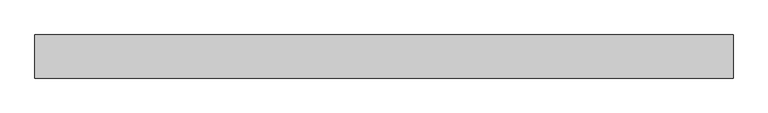
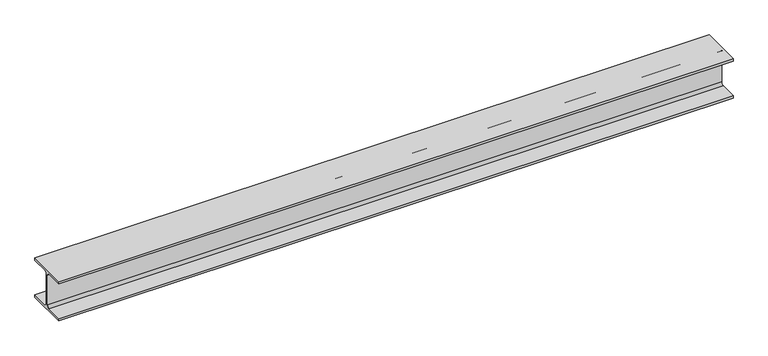
"""IFC4 building model written with IfcOpenShell, lengths in millimetres: beam geometry, 0912_Steel Framing_H-KSD3502 : H_SB_ASB_H-200x200x8x12."""

from ifc_helpers import new_model, si_unit, point, frame, frame_2d, origin, place, context, project, spatial, polyline, circle_curve, trimmed, segment, composite_curve, outline, extrude, source, transform, mapped, element, save


def beam_a703e86a(model_context):
    return source(origin(), model_context, "Body", "SweptSolid", [
        extrude(outline(composite_curve([segment(polyline([(100.0, -88.0), (100.0, -100.0), (-100.0, -100.0), (-100.0, -88.0), (-17.0, -88.0)]), True, "CONTINUOUS"), segment(trimmed(circle_curve(frame_2d((-17.0, -75.0)), 13.0), [point((-17.0, -88.0))], [point((-4.0, -75.0))], True, "CARTESIAN"), True, "CONTINUOUS"), segment(polyline([(-4.0, -75.0), (-4.0, 75.0)]), True, "CONTINUOUS"), segment(trimmed(circle_curve(frame_2d((-17.0, 75.0)), 13.0), [point((-4.0, 75.0))], [point((-17.0, 88.0))], True, "CARTESIAN"), True, "CONTINUOUS"), segment(polyline([(-17.0, 88.0), (-100.0, 88.0), (-100.0, 100.0), (100.0, 100.0), (100.0, 88.0), (17.0, 88.0)]), True, "CONTINUOUS"), segment(trimmed(circle_curve(frame_2d((17.0, 75.0)), 13.0), [point((17.0, 88.0))], [point((4.0, 75.0))], True, "CARTESIAN"), True, "CONTINUOUS"), segment(polyline([(4.0, 75.0), (4.0, -75.0)]), True, "CONTINUOUS"), segment(trimmed(circle_curve(frame_2d((17.0, -75.0)), 13.0), [point((4.0, -75.0))], [point((17.0, -88.0))], True, "CARTESIAN"), True, "CONTINUOUS"), segment(polyline([(17.0, -88.0), (100.0, -88.0)]), True, "CONTINUOUS")], self_intersect=False)), frame((-1414.4668129, 0.0, 0.0), z_axis=(1.0, 0.0, 0.0), x_axis=(0.0, 1.0, 0.0)), (0.0, 0.0, 1.0), 3240.4250908),
    ])


if __name__ == "__main__":
    model = new_model("IFC4")
    model_context = context("Model", 3, world=origin())
    ifc_project = project(units=[si_unit("LENGTHUNIT", "METRE", prefix="MILLI")], contexts=[model_context])
    site = spatial("IfcSite", under=ifc_project)
    building = spatial("IfcBuilding", under=site)
    placement = place(None, origin())
    beam_shape = beam_a703e86a(model_context)
    element("IfcBeam", 1, ObjectType="0912_Steel Framing_H-KSD3502 : H_SB_ASB_H-200x200x8x12", at=placement, inside=building, context=model_context, shape_type="MappedRepresentation", body=[
        mapped(beam_shape, transform((0.0, 0.0, 0.0), x_axis=(1.0, 0.0, 0.0), y_axis=(0.0, 1.0, 0.0), z_axis=(0.0, 0.0, 1.0))),
    ])
    save(model, "model.ifc")

# Revit data of these elements
# Type "0912_Steel Framing_H-KSD3502 : H_SB_ASB_H-200x200x8x12"
#   H_WM Code_1 = "S01AA002-00001 | Main Steel Structure Fabrication Work | Shelter/Building | Medium Steel - Standard (90KG/M>Weight≥30KG/M) | Material: (   )"
#   H_WM Code_2 = "S03AA028-00001 | Main Steel Structure Erection Work | Shelter/Building | Medium Steel (90KG/M>Weight≥30KG/M) | Material: (   )"
#   H_WM Code_3 = "S01AA010-00001 | Main Steel Structure Fabrication Work | Shelter/Building | Steel Painting/Coating | for Non-Fireproofed Steel Surface, Surface Preparation, Primer, Second & Final Coat | Material: (   )"
#   H_Q'ty Cal Type Tag = "SB-Q2"
#   Width = 20.0 cm
#   Web Thickness = 0.8 cm
#   Web Fillet = 1.3 cm
#   Warping Constant = 141000.0 cm⁶
#   W = 0
#   Torsional Moment of Inertia = 26.2485 cm⁴
#   Section Area = 63.53 cm²
#   Plastic Modulus weak axis = 244.0 cm³
#   Plastic Modulus strong axis = 525.0 cm³
#   Perimeter = 1.16 m²/m
#   Nominal Weight = 49.90 kgf/m
#   Moment of Inertia weak axis = 1600.00 cm⁴
#   Moment of Inertia strong axis = 4720.00 cm⁴
#   Height = 20.0 cm
#   Flange Thickness = 1.2 cm
#   Elastic Modulus weak axis = 160.0 cm³
#   Elastic Modulus strong axis = 472.0 cm³
#   Centroid Vertical = 10.0 cm
#   Centroid Horizontal = 10.0 cm
#   Ix = 47200000
#   Length [instance default] = 1.5240 m
#   Zx = 525000
#   b = 0.2000 m
#   h = 0.2000 m
#   r = 0.0130 m
#   s = 0.0080 m
#   t = 0.0120 m
#   A = 0.006353 m²
#   Structural Material [instance default] = Steel, 45-345
#   Assembly Code = ""
# Element 1 (IfcBeam, "0912_Steel Framing_H-KSD3502 : H_SB_ASB_H-200x200x8x12")
#   Structural Material = none
# Materials
#   "Steel, 45-345": class "Metal", colour RGB 189 187 185, transparency 0, Description = "Steel 345 MPa", Cost = 0
